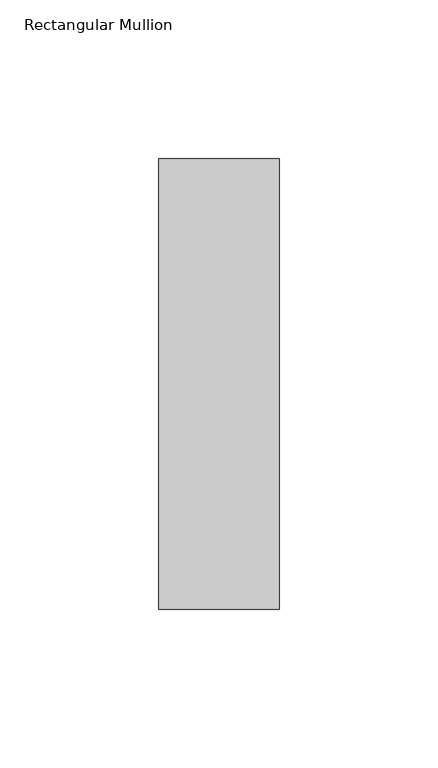
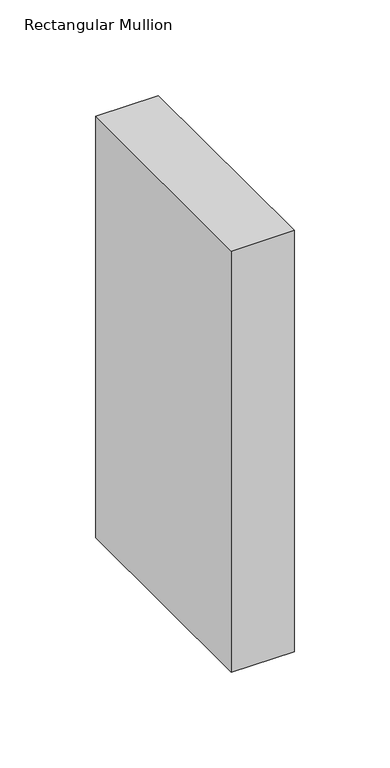
"""IFC4 building model written with IfcOpenShell, lengths in millimetres: member geometry, Rectangular Mullion : NLRS_21_CWM_hsb-regel 38x142_gen_rsf."""

from ifc_helpers import new_model, si_unit, frame, origin, place, context, project, spatial, polyline, outline, extrude, source, transform, mapped, element, save


def rectangular_mullion_ffaa0eaf(model_context):
    return source(origin(), model_context, "Body", "SweptSolid", [
        extrude(outline(polyline([(0.0, -71.0), (-38.0, -71.0), (-38.0, 71.0), (0.0, 71.0), (0.0, -71.0)])), frame((0.0, 0.0, -269.0000003), z_axis=(0.0, 0.0, 1.0), x_axis=(1.0, 0.0, 0.0)), (0.0, 0.0, 1.0), 269.0000003),
    ])


if __name__ == "__main__":
    model = new_model("IFC4")
    model_context = context("Model", 3, world=origin())
    ifc_project = project(units=[si_unit("LENGTHUNIT", "METRE", prefix="MILLI")], contexts=[model_context])
    site = spatial("IfcSite", under=ifc_project)
    building = spatial("IfcBuilding", under=site)
    placement = place(None, origin())
    rectangular_mullion_shape = rectangular_mullion_ffaa0eaf(model_context)
    element("IfcMember", 1, ObjectType="Rectangular Mullion : NLRS_21_CWM_hsb-regel 38x142_gen_rsf", at=placement, inside=building, context=model_context, shape_type="MappedRepresentation", body=[
        mapped(rectangular_mullion_shape, transform((0.0, 0.0, 0.0), x_axis=(1.0, 0.0, 0.0), y_axis=(0.0, 1.0, 0.0), z_axis=(0.0, 0.0, 1.0))),
    ])
    save(model, "model.ifc")

# Revit data of these elements
# Type "Rectangular Mullion : NLRS_21_CWM_hsb-regel 38x142_gen_rsf"
#   Export Type to IFC As = "IfcWall"
#   Type IfcGUID = "07M7mRoiH1CR8m_RSKIwpF"
#   Assembly Code = "21.10"
#   built-in parameter 1007322 = 0.465879 (stored number, unit not read)
#   built-in parameter 1007321 = 0.062336 (stored number, unit not read)
#   built-in parameter 1007320 = 0.062336 (stored number, unit not read)
# Element 1 (IfcMember, "Rectangular Mullion : NLRS_21_CWM_hsb-regel 38x142_gen_rsf")
#   Materials on its faces: "NLRS_i2_hout naaldhout vuren_gen_rsf"
# Materials
#   "NLRS_i2_hout naaldhout vuren_gen_rsf": class "I - Hout", colour RGB 234 199 147, transparency 0, Keynote = "i2", Manufacturer = "Revit Standards Foundation", URL = "www.revitstandards.org", Description = "hout vuren", Cost = 0
